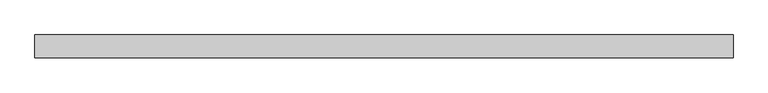
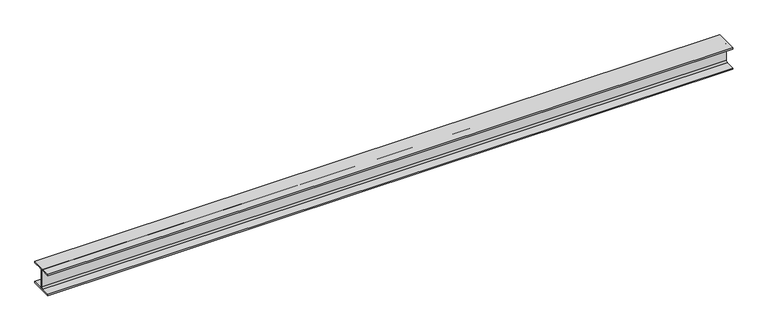
"""IFC4 building model written with IfcOpenShell, lengths in millimetres: beam geometry, 0912_Steel Framing_H-KSD3502 : H_SB_ASB_H-200x200x8x12."""

from ifc_helpers import new_model, si_unit, point, frame, frame_2d, origin, place, context, project, spatial, polyline, circle_curve, trimmed, segment, composite_curve, outline, extrude, source, transform, mapped, element, save


def beam_026c0679(model_context):
    return source(origin(), model_context, "Body", "SweptSolid", [
        extrude(outline(composite_curve([segment(polyline([(100.0, -88.0), (100.0, -100.0), (-100.0, -100.0), (-100.0, -88.0), (-17.0, -88.0)]), True, "CONTINUOUS"), segment(trimmed(circle_curve(frame_2d((-17.0, -75.0)), 13.0), [point((-17.0, -88.0))], [point((-4.0, -75.0))], True, "CARTESIAN"), True, "CONTINUOUS"), segment(polyline([(-4.0, -75.0), (-4.0, 75.0)]), True, "CONTINUOUS"), segment(trimmed(circle_curve(frame_2d((-17.0, 75.0)), 13.0), [point((-4.0, 75.0))], [point((-17.0, 88.0))], True, "CARTESIAN"), True, "CONTINUOUS"), segment(polyline([(-17.0, 88.0), (-100.0, 88.0), (-100.0, 100.0), (100.0, 100.0), (100.0, 88.0), (17.0, 88.0)]), True, "CONTINUOUS"), segment(trimmed(circle_curve(frame_2d((17.0, 75.0)), 13.0), [point((17.0, 88.0))], [point((4.0, 75.0))], True, "CARTESIAN"), True, "CONTINUOUS"), segment(polyline([(4.0, 75.0), (4.0, -75.0)]), True, "CONTINUOUS"), segment(trimmed(circle_curve(frame_2d((17.0, -75.0)), 13.0), [point((4.0, -75.0))], [point((17.0, -88.0))], True, "CARTESIAN"), True, "CONTINUOUS"), segment(polyline([(17.0, -88.0), (100.0, -88.0)]), True, "CONTINUOUS")], self_intersect=False)), frame((-3041.4802947, 0.0, 0.0), z_axis=(1.0, 0.0, 0.0), x_axis=(0.0, 1.0, 0.0)), (0.0, 0.0, 1.0), 6052.7309213),
    ])


if __name__ == "__main__":
    model = new_model("IFC4")
    model_context = context("Model", 3, world=origin())
    ifc_project = project(units=[si_unit("LENGTHUNIT", "METRE", prefix="MILLI")], contexts=[model_context])
    site = spatial("IfcSite", under=ifc_project)
    building = spatial("IfcBuilding", under=site)
    placement = place(None, origin())
    beam_shape = beam_026c0679(model_context)
    element("IfcBeam", 1, ObjectType="0912_Steel Framing_H-KSD3502 : H_SB_ASB_H-200x200x8x12", at=placement, inside=building, context=model_context, shape_type="MappedRepresentation", body=[
        mapped(beam_shape, transform((0.0, 0.0, 0.0), x_axis=(1.0, 0.0, 0.0), y_axis=(0.0, 1.0, 0.0), z_axis=(0.0, 0.0, 1.0))),
    ])
    save(model, "model.ifc")

# Revit data of these elements
# Type "0912_Steel Framing_H-KSD3502 : H_SB_ASB_H-200x200x8x12"
#   H_WM Code_1 = "S01AA002-00001 | Main Steel Structure Fabrication Work | Shelter/Building | Medium Steel - Standard (90KG/M>Weight≥30KG/M) | Material: (   )"
#   H_WM Code_2 = "S03AA028-00001 | Main Steel Structure Erection Work | Shelter/Building | Medium Steel (90KG/M>Weight≥30KG/M) | Material: (   )"
#   H_WM Code_3 = "S01AA010-00001 | Main Steel Structure Fabrication Work | Shelter/Building | Steel Painting/Coating | for Non-Fireproofed Steel Surface, Surface Preparation, Primer, Second & Final Coat | Material: (   )"
#   H_Q'ty Cal Type Tag = "SB-Q2"
#   Width = 20.0 cm
#   Web Thickness = 0.8 cm
#   Web Fillet = 1.3 cm
#   Warping Constant = 141000.0 cm⁶
#   W = 0
#   Torsional Moment of Inertia = 26.2485 cm⁴
#   Section Area = 63.53 cm²
#   Plastic Modulus weak axis = 244.0 cm³
#   Plastic Modulus strong axis = 525.0 cm³
#   Perimeter = 1.16 m²/m
#   Nominal Weight = 49.90 kgf/m
#   Moment of Inertia weak axis = 1600.00 cm⁴
#   Moment of Inertia strong axis = 4720.00 cm⁴
#   Height = 20.0 cm
#   Flange Thickness = 1.2 cm
#   Elastic Modulus weak axis = 160.0 cm³
#   Elastic Modulus strong axis = 472.0 cm³
#   Centroid Vertical = 10.0 cm
#   Centroid Horizontal = 10.0 cm
#   Ix = 47200000
#   Length [instance default] = 1.5240 m
#   Zx = 525000
#   b = 0.2000 m
#   h = 0.2000 m
#   r = 0.0130 m
#   s = 0.0080 m
#   t = 0.0120 m
#   A = 0.006353 m²
#   Structural Material [instance default] = Steel, 45-345
#   Assembly Code = ""
# Element 1 (IfcBeam, "0912_Steel Framing_H-KSD3502 : H_SB_ASB_H-200x200x8x12")
#   Structural Material = none
# Materials
#   "Steel, 45-345": class "Metal", colour RGB 189 187 185, transparency 0, Description = "Steel 345 MPa", Cost = 0
